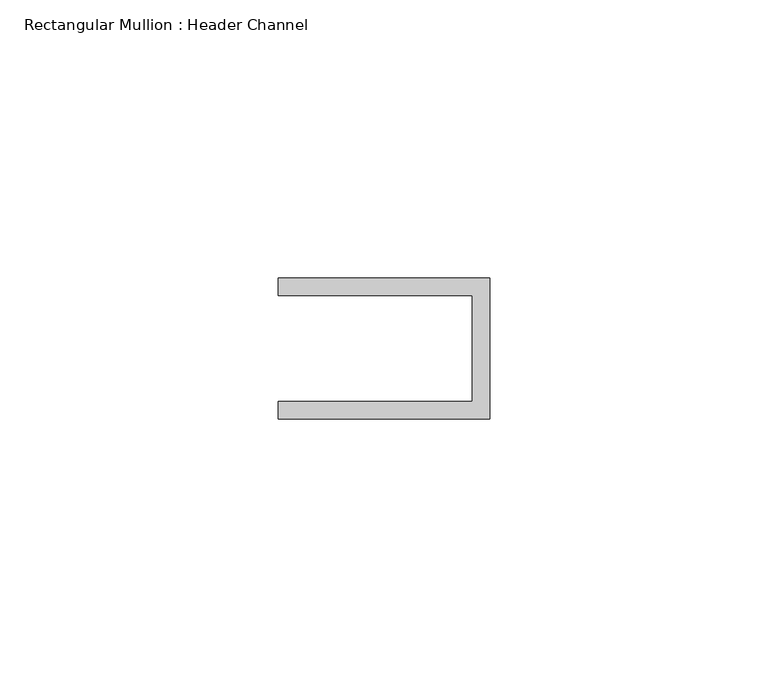
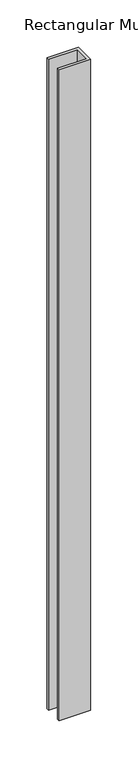
"""IFC4 building model written with IfcOpenShell, lengths in millimetres: member geometry, Rectangular Mullion : Header Channel."""

import ifcopenshell
import ifcopenshell.guid

model = None  # the IFC model being written
_history = None  # IfcOwnerHistory: only IFC2X3 demands one
_inside = {}  # id of a spatial element -> (the spatial element, [elements in it])
_under = {}  # id of a project, library or spatial element -> (it, [spatial elements below it])
_declared = {}  # id of a project -> (the project, [libraries it declares])
_typed = {}  # id of a type object -> (the type object, [elements of that type])
_made_of = {}  # id of a material, layer set ... -> (it, [elements and type objects made of it])


def new_model(schema):
    """Start an empty IFC model of exactly this schema.

    Asked for "IFC4X3", IfcOpenShell would pick the latest addendum, in which some entities
    have other attributes; the version numbers below select the first issue.
    IFC2X3 requires an IfcOwnerHistory on every rooted entity: one is made here for all.
    """
    global model, _history
    if schema == "IFC4X3":
        model = ifcopenshell.file(schema_version=(4, 3, 0, 0))
    else:
        model = ifcopenshell.file(schema=schema)
    _inside.clear()
    _under.clear()
    _declared.clear()
    _typed.clear()
    _made_of.clear()
    _history = None
    if model.schema == "IFC2X3":
        org = make("IfcOrganization", Name="unknown")
        user = make(
            "IfcPersonAndOrganization",
            ThePerson=make("IfcPerson", FamilyName="unknown"),
            TheOrganization=org,
        )
        app = make(
            "IfcApplication",
            ApplicationDeveloper=org,
            Version="unknown",
            ApplicationFullName="unknown",
            ApplicationIdentifier="unknown",
        )
        _history = make(
            "IfcOwnerHistory",
            OwningUser=user,
            OwningApplication=app,
            ChangeAction="ADDED",
            CreationDate=0,
        )
    return model


def make(cls, **values):
    """One entity of the class cls with the attributes given. An attribute that is None is left unset."""
    return model.create_entity(
        cls, **{name: value for name, value in values.items() if value is not None}
    )


def rooted(cls, **values):
    """An entity with a GlobalId (a new one), such as an element, a storey or a relation."""
    return make(cls, GlobalId=ifcopenshell.guid.new(), OwnerHistory=_history, **values)


def si_unit(unit_type, name, prefix=None):
    """IfcSIUnit, for example si_unit("LENGTHUNIT", "METRE", prefix="MILLI")."""
    return make("IfcSIUnit", UnitType=unit_type, Prefix=prefix, Name=name)


def assignment(units):
    """IfcUnitAssignment: the units of a project."""
    return None if units is None else make("IfcUnitAssignment", Units=units)


def point(xyz):
    """IfcCartesianPoint."""
    return None if xyz is None else make("IfcCartesianPoint", Coordinates=xyz)


def direction(xyz):
    """IfcDirection."""
    return None if xyz is None else make("IfcDirection", DirectionRatios=xyz)


def frame(location, z_axis=None, x_axis=None):
    """IfcAxis2Placement3D, a coordinate frame: its origin and axes. An axis left out is left unset."""
    return make(
        "IfcAxis2Placement3D",
        Location=point(location),
        Axis=direction(z_axis),
        RefDirection=direction(x_axis),
    )


def origin():
    """The frame at (0, 0, 0) with its axes left unset."""
    return frame((0.0, 0.0, 0.0))


def place(relative_to, where):
    """IfcLocalPlacement: puts the frame where relative to a parent placement (None: the world)."""
    return make(
        "IfcLocalPlacement", PlacementRelTo=relative_to, RelativePlacement=where
    )


def context(
    kind, dimensions, precision=None, world=None, true_north=None, identifier=None
):
    """IfcGeometricRepresentationContext, for example the 3D "Model" context."""
    return make(
        "IfcGeometricRepresentationContext",
        ContextIdentifier=identifier,
        ContextType=kind,
        CoordinateSpaceDimension=dimensions,
        Precision=precision,
        WorldCoordinateSystem=world,
        TrueNorth=true_north,
    )


def project(units=None, contexts=None):
    """IfcProject with its units and contexts."""
    return rooted(
        "IfcProject",
        Name="project",
        RepresentationContexts=contexts,
        UnitsInContext=assignment(units),
    )


def spatial(cls, under=None, at=None, **own):
    """A site, building, storey or space (cls), placed at a placement, below another one or the project."""
    s = rooted(cls, ObjectPlacement=at, **own)
    if under is not None:
        _under.setdefault(under.id(), (under, []))[1].append(s)
    return s


def polyline(points):
    """IfcPolyline through the points."""
    return make("IfcPolyline", Points=[point(p) for p in points])


def outline(outer, holes=None, kind="AREA"):
    """IfcArbitraryClosedProfileDef: a profile drawn as a closed curve; with holes, ...WithVoids."""
    if holes is None:
        return make("IfcArbitraryClosedProfileDef", ProfileType=kind, OuterCurve=outer)
    return make(
        "IfcArbitraryProfileDefWithVoids",
        ProfileType=kind,
        OuterCurve=outer,
        InnerCurves=holes,
    )


def extrude(swept, where, along, depth):
    """IfcExtrudedAreaSolid: the profile swept, set in the frame where, extruded along a direction by depth."""
    return make(
        "IfcExtrudedAreaSolid",
        SweptArea=swept,
        Position=where,
        ExtrudedDirection=direction(along),
        Depth=depth,
    )


def shape(context_of_items, identifier, shape_type, items):
    """IfcShapeRepresentation: the items that make up one representation, for example the "Body"."""
    return make(
        "IfcShapeRepresentation",
        ContextOfItems=context_of_items,
        RepresentationIdentifier=identifier,
        RepresentationType=shape_type,
        Items=items,
    )


def source(mapping_origin, context_of_items, identifier, shape_type, items):
    """IfcRepresentationMap: a shape defined once, which mapped items show again and again."""
    return make(
        "IfcRepresentationMap",
        MappingOrigin=mapping_origin,
        MappedRepresentation=shape(context_of_items, identifier, shape_type, items),
    )


def transform(
    local_origin,
    x_axis=None,
    y_axis=None,
    z_axis=None,
    scale=None,
    scale2=None,
    scale3=None,
    uniform=True,
):
    """IfcCartesianTransformationOperator3D, or its non-uniform kind. x_axis, y_axis, z_axis: its Axis1, 2, 3."""
    if uniform:
        return make(
            "IfcCartesianTransformationOperator3D",
            Axis1=direction(x_axis),
            Axis2=direction(y_axis),
            LocalOrigin=point(local_origin),
            Scale=scale,
            Axis3=direction(z_axis),
        )
    return make(
        "IfcCartesianTransformationOperator3DnonUniform",
        Axis1=direction(x_axis),
        Axis2=direction(y_axis),
        LocalOrigin=point(local_origin),
        Scale=scale,
        Axis3=direction(z_axis),
        Scale2=scale2,
        Scale3=scale3,
    )


def mapped(mapping_source, mapping_target):
    """IfcMappedItem: shows the shape of a source again, moved by a transform."""
    return make(
        "IfcMappedItem", MappingSource=mapping_source, MappingTarget=mapping_target
    )


def made_of(thing, what):
    """Note that an element or type object is made of a material, layer set ...; save() writes the relation."""
    if what is not None:
        _made_of.setdefault(what.id(), (what, []))[1].append(thing)
    return thing


def element(
    cls,
    number,
    at=None,
    inside=None,
    cuts=None,
    type_object=None,
    material=None,
    context=None,
    identifier="Body",
    shape_type=None,
    held_by="IfcProductDefinitionShape",
    body=None,
    shapes=None,
    **own,
):
    """One element of the class cls, such as IfcWall. Its Tag is "e" and its number.

    at: its placement. inside: the storey or other place that contains it. cuts: it is an
    opening in that element (IfcRelVoidsElement). A single representation is given by context,
    identifier, shape_type and body (its items); several are given by shapes. held_by: the class
    of the entity that holds the representations. save() writes the other relations.
    """
    e = rooted(cls, Tag="e%d" % number, ObjectPlacement=at, **own)
    if body is not None:
        shapes = [shape(context, identifier, shape_type, body)]
    if shapes is not None:
        e.Representation = make(held_by, Representations=shapes)
    if inside is not None:
        _inside.setdefault(inside.id(), (inside, []))[1].append(e)
    if cuts is not None:
        rooted(
            "IfcRelVoidsElement", RelatingBuildingElement=cuts, RelatedOpeningElement=e
        )
    if type_object is not None:
        _typed.setdefault(type_object.id(), (type_object, []))[1].append(e)
    return made_of(e, material)


def aggregate(whole, parts):
    """IfcRelAggregates: a whole, such as a stair, and the parts it consists of."""
    return rooted("IfcRelAggregates", RelatingObject=whole, RelatedObjects=parts)


def save(model, path):
    """Write the relations noted so far, then the file.

    IfcRelAggregates (storeys below a building ...), IfcRelContainedInSpatialStructure (elements
    in a storey), IfcRelDefinesByType, IfcRelAssociatesMaterial and IfcRelDeclares: one each for
    every whole, place, type object, material and project.
    """
    for whole, parts in _under.values():
        aggregate(whole, parts)
    for where, things in _inside.values():
        rooted(
            "IfcRelContainedInSpatialStructure",
            RelatedElements=things,
            RelatingStructure=where,
        )
    for kind, things in _typed.values():
        rooted("IfcRelDefinesByType", RelatedObjects=things, RelatingType=kind)
    for what, things in _made_of.values():
        rooted("IfcRelAssociatesMaterial", RelatedObjects=things, RelatingMaterial=what)
    for by, libraries in _declared.values():
        rooted("IfcRelDeclares", RelatingContext=by, RelatedDefinitions=libraries)
    model.write(path)


def rectangular_mullion_header_channel_ba5daf2f(model_context):
    return source(origin(), model_context, "Body", "SweptSolid", [
        extrude(outline(polyline([(0.0, -12.7), (-38.1, -12.7), (-38.1, -9.525), (-3.175, -9.525), (-3.175, 9.525), (-38.1, 9.525), (-38.1, 12.7), (0.0, 12.7), (0.0, -12.7)])), frame((0.0, 0.0, -838.2000002), z_axis=(0.0, 0.0, 1.0), x_axis=(1.0, 0.0, 0.0)), (0.0, 0.0, 1.0), 838.2000002),
    ])


if __name__ == "__main__":
    model = new_model("IFC4")
    model_context = context("Model", 3, world=origin())
    ifc_project = project(units=[si_unit("LENGTHUNIT", "METRE", prefix="MILLI")], contexts=[model_context])
    site = spatial("IfcSite", under=ifc_project)
    building = spatial("IfcBuilding", under=site)
    placement = place(None, origin())
    rectangular_mullion_header_channel_shape = rectangular_mullion_header_channel_ba5daf2f(model_context)
    element("IfcMember", 1, ObjectType="Rectangular Mullion : Header Channel", at=placement, inside=building, context=model_context, shape_type="MappedRepresentation", body=[
        mapped(rectangular_mullion_header_channel_shape, transform((0.0, 0.0, 0.0), x_axis=(1.0, 0.0, 0.0), y_axis=(0.0, 1.0, 0.0), z_axis=(0.0, 0.0, 1.0))),
    ])
    save(model, "model.ifc")

# Revit data of these elements
# Type "Rectangular Mullion : Header Channel"
#   built-in parameter 1007322 = 0.0833333 (stored number, unit not read)
#   built-in parameter 1007321 = -0.03125 (stored number, unit not read)
#   built-in parameter 1007320 = 0.0416667 (stored number, unit not read)
# Element 1 (IfcMember, "Rectangular Mullion : Header Channel")
#   Materials on its faces: "ALUM"
# Materials
#   "ALUM": class "Generic", colour RGB 157 157 157, transparency 0, Cost = 0
